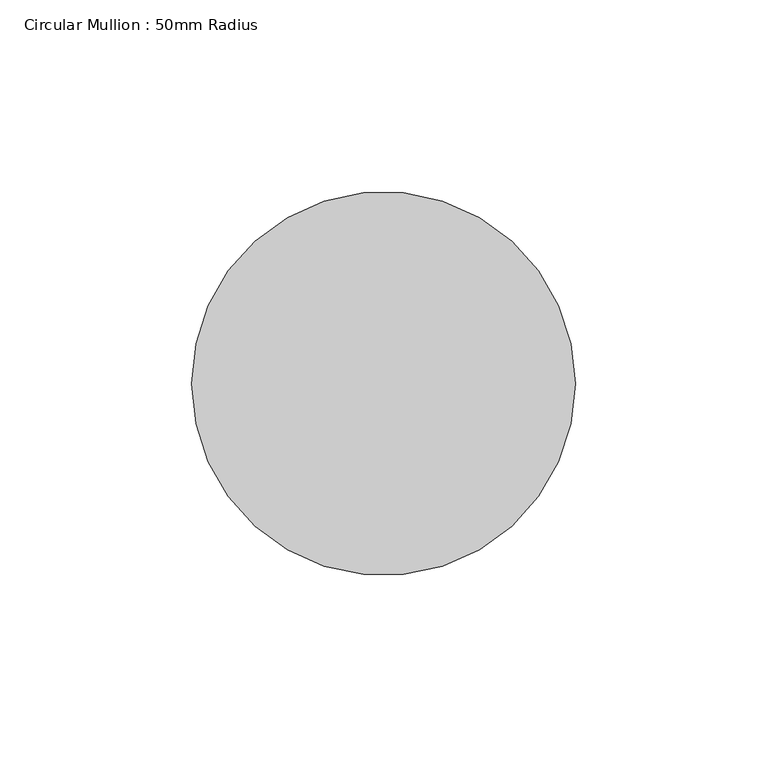
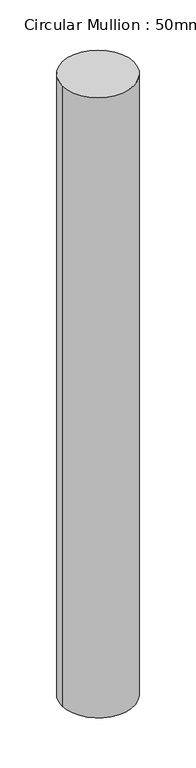
"""IFC4 building model written with IfcOpenShell, lengths in millimetres: member geometry, Circular Mullion : 50mm Radius."""

from ifc_helpers import new_model, si_unit, point, frame, origin, origin_2d, place, context, project, spatial, circle_curve, trimmed, segment, composite_curve, outline, extrude, source, transform, mapped, element, save


def circular_mullion_50mm_radius_4a922d1c(model_context):
    return source(origin(), model_context, "Body", "SweptSolid", [
        extrude(outline(composite_curve([segment(trimmed(circle_curve(origin_2d(), 50.0), [point((50.0, 0.0))], [point((-50.0, 0.0))], False, "CARTESIAN"), True, "CONTINUOUS"), segment(trimmed(circle_curve(origin_2d(), 50.0), [point((-50.0, 0.0))], [point((50.0, 0.0))], False, "CARTESIAN"), True, "CONTINUOUS")], self_intersect=False)), frame((0.0, 0.0, -914.4221189), z_axis=(0.0, 0.0, 1.0), x_axis=(1.0, 0.0, 0.0)), (0.0, 0.0, 1.0), 914.4221189),
    ])


if __name__ == "__main__":
    model = new_model("IFC4")
    model_context = context("Model", 3, world=origin())
    ifc_project = project(units=[si_unit("LENGTHUNIT", "METRE", prefix="MILLI")], contexts=[model_context])
    site = spatial("IfcSite", under=ifc_project)
    building = spatial("IfcBuilding", under=site)
    placement = place(None, origin())
    circular_mullion_50mm_radius_shape = circular_mullion_50mm_radius_4a922d1c(model_context)
    element("IfcMember", 1, ObjectType="Circular Mullion : 50mm Radius", at=placement, inside=building, context=model_context, shape_type="MappedRepresentation", body=[
        mapped(circular_mullion_50mm_radius_shape, transform((0.0, 0.0, 0.0), x_axis=(1.0, 0.0, 0.0), y_axis=(0.0, 1.0, 0.0), z_axis=(0.0, 0.0, 1.0))),
    ])
    save(model, "model.ifc")

# Revit data of these elements
# Type "Circular Mullion : 50mm Radius"
#   built-in parameter 1007350 = 0.164042 (stored number, unit not read)
# Element 1 (IfcMember, "Circular Mullion : 50mm Radius")
#   Materials on its faces: "Aluminium"
# Materials
#   "Aluminium": class "Metal", colour RGB 247 247 247, transparency 0, Description = "Aluminium 6061", Cost = 0
